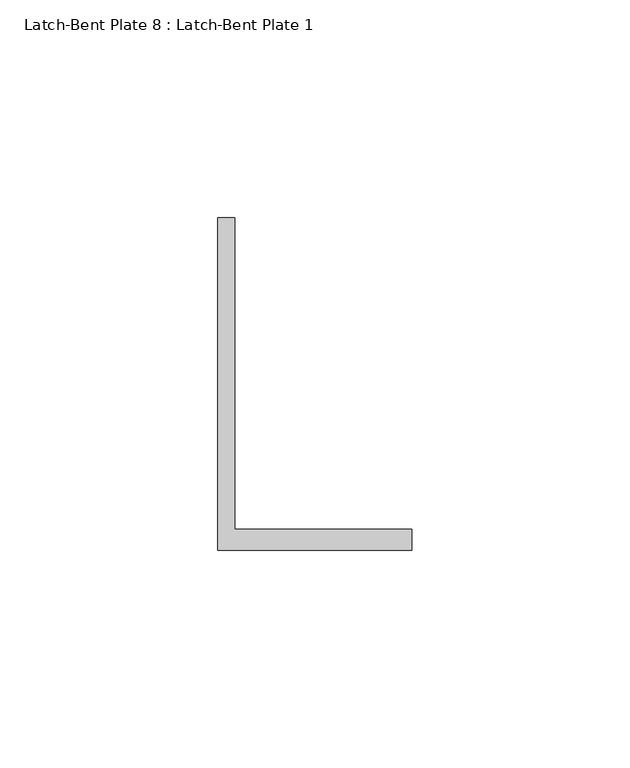
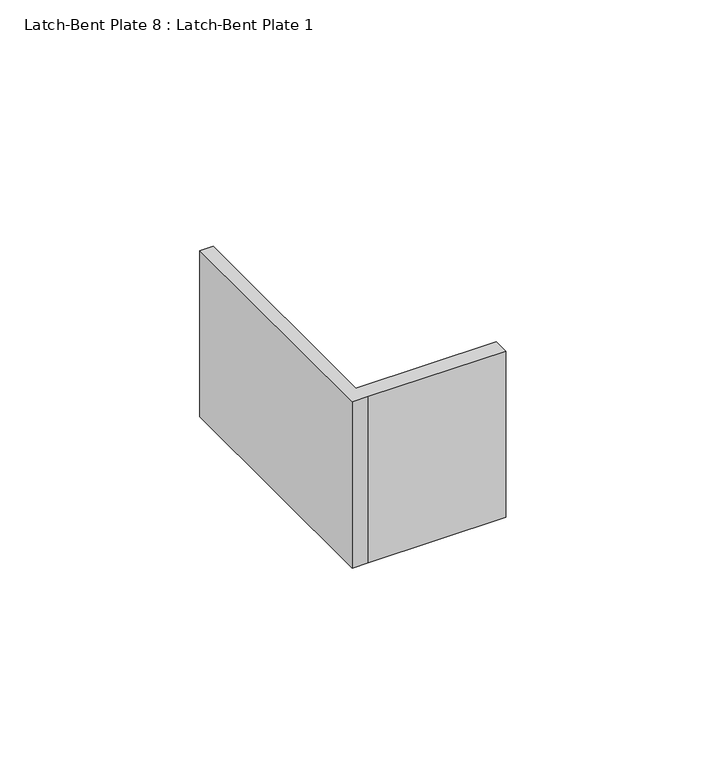
"""IFC4 building model written with IfcOpenShell, lengths in millimetres: proxy geometry, Latch-Bent Plate 8 : Latch-Bent Plate 1."""

from ifc_helpers import new_model, si_unit, frame, origin, place, context, project, spatial, polyline, outline, extrude, source, transform, mapped, element, save


def latch_bent_plate_8_latch_bent_plate_1_71f9beff(model_context):
    return source(origin(), model_context, "Body", "SweptSolid", [
        extrude(outline(polyline([(587327.0060739, -532877.4663841), (587322.2435739, -532877.4663841), (587322.2435739, -532801.2663841), (587326.1141748, -532801.2663841), (587326.1141748, -532872.7038841), (587366.6808739, -532872.7038841), (587366.6808739, -532877.4663841), (587327.0060739, -532877.4663841)])), frame((0.0, 0.0, 1041.4), z_axis=(0.0, 0.0, 1.0), x_axis=(1.0, 0.0, 0.0)), (0.0, 0.0, 1.0), 50.8),
    ])


if __name__ == "__main__":
    model = new_model("IFC4")
    model_context = context("Model", 3, world=origin())
    ifc_project = project(units=[si_unit("LENGTHUNIT", "METRE", prefix="MILLI")], contexts=[model_context])
    site = spatial("IfcSite", under=ifc_project)
    building = spatial("IfcBuilding", under=site)
    placement = place(None, origin())
    latch_bent_plate_8_latch_bent_plate_1_shape = latch_bent_plate_8_latch_bent_plate_1_71f9beff(model_context)
    element("IfcBuildingElementProxy", 1, Name="Latch-Bent Plate 8 : Latch-Bent Plate 1", ObjectType="Latch-Bent Plate 8 : Latch-Bent Plate 1", at=placement, inside=building, context=model_context, shape_type="MappedRepresentation", body=[
        mapped(latch_bent_plate_8_latch_bent_plate_1_shape, transform((0.0, 0.0, 0.0), x_axis=(1.0, 0.0, 0.0), y_axis=(0.0, 1.0, 0.0), z_axis=(0.0, 0.0, 1.0))),
    ])
    save(model, "model.ifc")

# Revit data of these elements
# Element 1 (IfcBuildingElementProxy, "Latch-Bent Plate 8 : Latch-Bent Plate 1")
#   Materials on its faces: "GALV. GATE LATCH"
# Materials
#   "GALV. GATE LATCH": class "Metal", colour RGB 189 187 185, transparency 0, Description = "Carbon steel", Cost = 0
